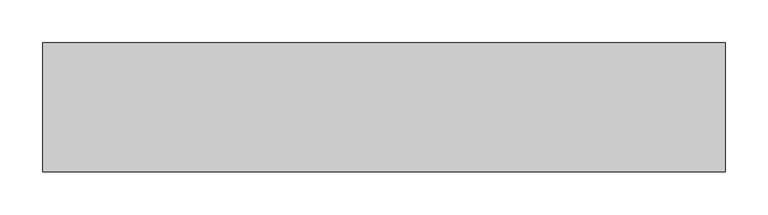
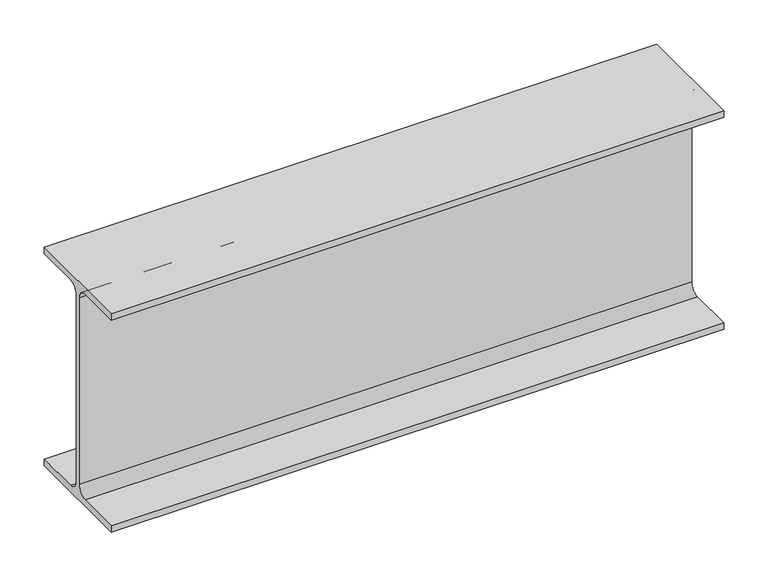
"""IFC4 building model written with IfcOpenShell, lengths in millimetres: beam geometry, 0912_Steel Framing_H-KSD3502 : H_SB_ASB_H-300x150x6.5x9."""

from ifc_helpers import new_model, si_unit, point, frame, frame_2d, origin, place, context, project, spatial, polyline, circle_curve, trimmed, segment, composite_curve, outline, extrude, source, transform, mapped, element, save


def beam_e2def3fa(model_context):
    return source(origin(), model_context, "Body", "SweptSolid", [
        extrude(outline(composite_curve([segment(polyline([(75.0, -141.0), (75.0, -150.0), (-75.0, -150.0), (-75.0, -141.0), (-16.25, -141.0)]), True, "CONTINUOUS"), segment(trimmed(circle_curve(frame_2d((-16.25, -128.0)), 13.0), [point((-16.25, -141.0))], [point((-3.25, -128.0))], True, "CARTESIAN"), True, "CONTINUOUS"), segment(polyline([(-3.25, -128.0), (-3.25, 128.0)]), True, "CONTINUOUS"), segment(trimmed(circle_curve(frame_2d((-16.25, 128.0)), 13.0), [point((-3.25, 128.0))], [point((-16.25, 141.0))], True, "CARTESIAN"), True, "CONTINUOUS"), segment(polyline([(-16.25, 141.0), (-75.0, 141.0), (-75.0, 150.0), (75.0, 150.0), (75.0, 141.0), (16.25, 141.0)]), True, "CONTINUOUS"), segment(trimmed(circle_curve(frame_2d((16.25, 128.0)), 13.0), [point((16.25, 141.0))], [point((3.25, 128.0))], True, "CARTESIAN"), True, "CONTINUOUS"), segment(polyline([(3.25, 128.0), (3.25, -128.0)]), True, "CONTINUOUS"), segment(trimmed(circle_curve(frame_2d((16.25, -128.0)), 13.0), [point((3.25, -128.0))], [point((16.25, -141.0))], True, "CARTESIAN"), True, "CONTINUOUS"), segment(polyline([(16.25, -141.0), (75.0, -141.0)]), True, "CONTINUOUS")], self_intersect=False)), frame((-445.0, 0.0, 0.0), z_axis=(1.0, 0.0, 0.0), x_axis=(0.0, 1.0, 0.0)), (0.0, 0.0, 1.0), 794.8),
    ])


if __name__ == "__main__":
    model = new_model("IFC4")
    model_context = context("Model", 3, world=origin())
    ifc_project = project(units=[si_unit("LENGTHUNIT", "METRE", prefix="MILLI")], contexts=[model_context])
    site = spatial("IfcSite", under=ifc_project)
    building = spatial("IfcBuilding", under=site)
    placement = place(None, origin())
    beam_shape = beam_e2def3fa(model_context)
    element("IfcBeam", 1, ObjectType="0912_Steel Framing_H-KSD3502 : H_SB_ASB_H-300x150x6.5x9", at=placement, inside=building, context=model_context, shape_type="MappedRepresentation", body=[
        mapped(beam_shape, transform((0.0, 0.0, 0.0), x_axis=(1.0, 0.0, 0.0), y_axis=(0.0, 1.0, 0.0), z_axis=(0.0, 0.0, 1.0))),
    ])
    save(model, "model.ifc")

# Revit data of these elements
# Type "0912_Steel Framing_H-KSD3502 : H_SB_ASB_H-300x150x6.5x9"
#   H_WM Code_1 = "S01AA002-00001 | Main Steel Structure Fabrication Work | Shelter/Building | Medium Steel - Standard (90KG/M>Weight≥30KG/M) | Material: (   )"
#   H_WM Code_2 = "S03AA028-00001 | Main Steel Structure Erection Work | Shelter/Building | Medium Steel (90KG/M>Weight≥30KG/M) | Material: (   )"
#   H_WM Code_3 = "S01AA010-00001 | Main Steel Structure Fabrication Work | Shelter/Building | Steel Painting/Coating | for Non-Fireproofed Steel Surface, Surface Preparation, Primer, Second & Final Coat | Material: (   )"
#   H_Q'ty Cal Type Tag = "SB-Q2"
#   Width = 15.0 cm
#   Web Thickness = 0.65 cm
#   Web Fillet = 1.3 cm
#   Warping Constant = 107000.0 cm⁶
#   W = 0
#   Torsional Moment of Inertia = 9.9539 cm⁴
#   Section Area = 46.78 cm²
#   Plastic Modulus weak axis = 105.0 cm³
#   Plastic Modulus strong axis = 542.0 cm³
#   Perimeter = 1.17 m²/m
#   Nominal Weight = 36.70 kgf/m
#   Moment of Inertia weak axis = 508.00 cm⁴
#   Moment of Inertia strong axis = 7210.00 cm⁴
#   Height = 30.0 cm
#   Flange Thickness = 0.9 cm
#   Elastic Modulus weak axis = 67.7 cm³
#   Elastic Modulus strong axis = 481.0 cm³
#   Centroid Vertical = 15.0 cm
#   Centroid Horizontal = 7.5 cm
#   Ix = 72100000
#   Length [instance default] = 1.5240 m
#   Zx = 542000
#   b = 0.1500 m
#   h = 0.3000 m
#   r = 0.0130 m
#   s = 0.0065 m
#   t = 0.0090 m
#   A = 0.004678 m²
#   Structural Material [instance default] = Steel, 45-345
#   Assembly Code = ""
# Element 1 (IfcBeam, "0912_Steel Framing_H-KSD3502 : H_SB_ASB_H-300x150x6.5x9")
#   Structural Material = none
# Materials
#   "Steel, 45-345": class "Metal", colour RGB 189 187 185, transparency 0, Description = "Steel 345 MPa", Cost = 0
